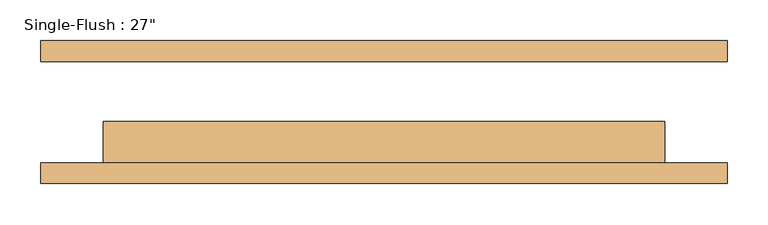
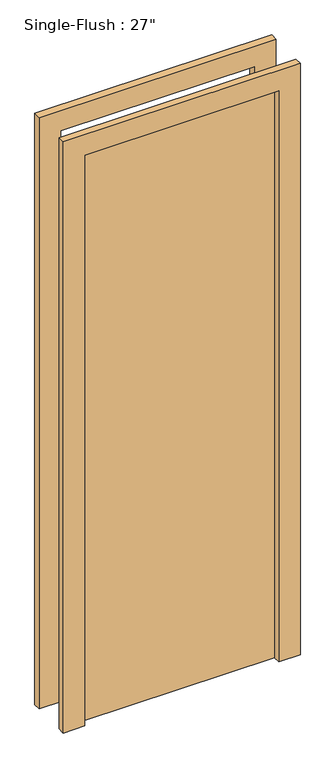
"""IFC4 building model written with IfcOpenShell, lengths in millimetres: door geometry."""

import ifcopenshell
import ifcopenshell.guid

model = None  # the IFC model being written
_history = None  # IfcOwnerHistory: only IFC2X3 demands one
_inside = {}  # id of a spatial element -> (the spatial element, [elements in it])
_under = {}  # id of a project, library or spatial element -> (it, [spatial elements below it])
_declared = {}  # id of a project -> (the project, [libraries it declares])
_typed = {}  # id of a type object -> (the type object, [elements of that type])
_made_of = {}  # id of a material, layer set ... -> (it, [elements and type objects made of it])


def new_model(schema):
    """Start an empty IFC model of exactly this schema.

    Asked for "IFC4X3", IfcOpenShell would pick the latest addendum, in which some entities
    have other attributes; the version numbers below select the first issue.
    IFC2X3 requires an IfcOwnerHistory on every rooted entity: one is made here for all.
    """
    global model, _history
    if schema == "IFC4X3":
        model = ifcopenshell.file(schema_version=(4, 3, 0, 0))
    else:
        model = ifcopenshell.file(schema=schema)
    _inside.clear()
    _under.clear()
    _declared.clear()
    _typed.clear()
    _made_of.clear()
    _history = None
    if model.schema == "IFC2X3":
        org = make("IfcOrganization", Name="unknown")
        user = make(
            "IfcPersonAndOrganization",
            ThePerson=make("IfcPerson", FamilyName="unknown"),
            TheOrganization=org,
        )
        app = make(
            "IfcApplication",
            ApplicationDeveloper=org,
            Version="unknown",
            ApplicationFullName="unknown",
            ApplicationIdentifier="unknown",
        )
        _history = make(
            "IfcOwnerHistory",
            OwningUser=user,
            OwningApplication=app,
            ChangeAction="ADDED",
            CreationDate=0,
        )
    return model


def make(cls, **values):
    """One entity of the class cls with the attributes given. An attribute that is None is left unset."""
    return model.create_entity(
        cls, **{name: value for name, value in values.items() if value is not None}
    )


def rooted(cls, **values):
    """An entity with a GlobalId (a new one), such as an element, a storey or a relation."""
    return make(cls, GlobalId=ifcopenshell.guid.new(), OwnerHistory=_history, **values)


def si_unit(unit_type, name, prefix=None):
    """IfcSIUnit, for example si_unit("LENGTHUNIT", "METRE", prefix="MILLI")."""
    return make("IfcSIUnit", UnitType=unit_type, Prefix=prefix, Name=name)


def assignment(units):
    """IfcUnitAssignment: the units of a project."""
    return None if units is None else make("IfcUnitAssignment", Units=units)


def point(xyz):
    """IfcCartesianPoint."""
    return None if xyz is None else make("IfcCartesianPoint", Coordinates=xyz)


def direction(xyz):
    """IfcDirection."""
    return None if xyz is None else make("IfcDirection", DirectionRatios=xyz)


def frame(location, z_axis=None, x_axis=None):
    """IfcAxis2Placement3D, a coordinate frame: its origin and axes. An axis left out is left unset."""
    return make(
        "IfcAxis2Placement3D",
        Location=point(location),
        Axis=direction(z_axis),
        RefDirection=direction(x_axis),
    )


def origin():
    """The frame at (0, 0, 0) with its axes left unset."""
    return frame((0.0, 0.0, 0.0))


def origin_with_axes():
    """The frame at (0, 0, 0) with the z axis (0, 0, 1) and the x axis (1, 0, 0) written out."""
    return frame((0.0, 0.0, 0.0), z_axis=(0.0, 0.0, 1.0), x_axis=(1.0, 0.0, 0.0))


def place(relative_to, where):
    """IfcLocalPlacement: puts the frame where relative to a parent placement (None: the world)."""
    return make(
        "IfcLocalPlacement", PlacementRelTo=relative_to, RelativePlacement=where
    )


def context(
    kind, dimensions, precision=None, world=None, true_north=None, identifier=None
):
    """IfcGeometricRepresentationContext, for example the 3D "Model" context."""
    return make(
        "IfcGeometricRepresentationContext",
        ContextIdentifier=identifier,
        ContextType=kind,
        CoordinateSpaceDimension=dimensions,
        Precision=precision,
        WorldCoordinateSystem=world,
        TrueNorth=true_north,
    )


def project(units=None, contexts=None):
    """IfcProject with its units and contexts."""
    return rooted(
        "IfcProject",
        Name="project",
        RepresentationContexts=contexts,
        UnitsInContext=assignment(units),
    )


def spatial(cls, under=None, at=None, **own):
    """A site, building, storey or space (cls), placed at a placement, below another one or the project."""
    s = rooted(cls, ObjectPlacement=at, **own)
    if under is not None:
        _under.setdefault(under.id(), (under, []))[1].append(s)
    return s


def polyline(points):
    """IfcPolyline through the points."""
    return make("IfcPolyline", Points=[point(p) for p in points])


def outline(outer, holes=None, kind="AREA"):
    """IfcArbitraryClosedProfileDef: a profile drawn as a closed curve; with holes, ...WithVoids."""
    if holes is None:
        return make("IfcArbitraryClosedProfileDef", ProfileType=kind, OuterCurve=outer)
    return make(
        "IfcArbitraryProfileDefWithVoids",
        ProfileType=kind,
        OuterCurve=outer,
        InnerCurves=holes,
    )


def extrude(swept, where, along, depth):
    """IfcExtrudedAreaSolid: the profile swept, set in the frame where, extruded along a direction by depth."""
    return make(
        "IfcExtrudedAreaSolid",
        SweptArea=swept,
        Position=where,
        ExtrudedDirection=direction(along),
        Depth=depth,
    )


def shape(context_of_items, identifier, shape_type, items):
    """IfcShapeRepresentation: the items that make up one representation, for example the "Body"."""
    return make(
        "IfcShapeRepresentation",
        ContextOfItems=context_of_items,
        RepresentationIdentifier=identifier,
        RepresentationType=shape_type,
        Items=items,
    )


def source(mapping_origin, context_of_items, identifier, shape_type, items):
    """IfcRepresentationMap: a shape defined once, which mapped items show again and again."""
    return make(
        "IfcRepresentationMap",
        MappingOrigin=mapping_origin,
        MappedRepresentation=shape(context_of_items, identifier, shape_type, items),
    )


def transform(
    local_origin,
    x_axis=None,
    y_axis=None,
    z_axis=None,
    scale=None,
    scale2=None,
    scale3=None,
    uniform=True,
):
    """IfcCartesianTransformationOperator3D, or its non-uniform kind. x_axis, y_axis, z_axis: its Axis1, 2, 3."""
    if uniform:
        return make(
            "IfcCartesianTransformationOperator3D",
            Axis1=direction(x_axis),
            Axis2=direction(y_axis),
            LocalOrigin=point(local_origin),
            Scale=scale,
            Axis3=direction(z_axis),
        )
    return make(
        "IfcCartesianTransformationOperator3DnonUniform",
        Axis1=direction(x_axis),
        Axis2=direction(y_axis),
        LocalOrigin=point(local_origin),
        Scale=scale,
        Axis3=direction(z_axis),
        Scale2=scale2,
        Scale3=scale3,
    )


def mapped(mapping_source, mapping_target):
    """IfcMappedItem: shows the shape of a source again, moved by a transform."""
    return make(
        "IfcMappedItem", MappingSource=mapping_source, MappingTarget=mapping_target
    )


def made_of(thing, what):
    """Note that an element or type object is made of a material, layer set ...; save() writes the relation."""
    if what is not None:
        _made_of.setdefault(what.id(), (what, []))[1].append(thing)
    return thing


def element(
    cls,
    number,
    at=None,
    inside=None,
    cuts=None,
    type_object=None,
    material=None,
    context=None,
    identifier="Body",
    shape_type=None,
    held_by="IfcProductDefinitionShape",
    body=None,
    shapes=None,
    **own,
):
    """One element of the class cls, such as IfcWall. Its Tag is "e" and its number.

    at: its placement. inside: the storey or other place that contains it. cuts: it is an
    opening in that element (IfcRelVoidsElement). A single representation is given by context,
    identifier, shape_type and body (its items); several are given by shapes. held_by: the class
    of the entity that holds the representations. save() writes the other relations.
    """
    e = rooted(cls, Tag="e%d" % number, ObjectPlacement=at, **own)
    if body is not None:
        shapes = [shape(context, identifier, shape_type, body)]
    if shapes is not None:
        e.Representation = make(held_by, Representations=shapes)
    if inside is not None:
        _inside.setdefault(inside.id(), (inside, []))[1].append(e)
    if cuts is not None:
        rooted(
            "IfcRelVoidsElement", RelatingBuildingElement=cuts, RelatedOpeningElement=e
        )
    if type_object is not None:
        _typed.setdefault(type_object.id(), (type_object, []))[1].append(e)
    return made_of(e, material)


def aggregate(whole, parts):
    """IfcRelAggregates: a whole, such as a stair, and the parts it consists of."""
    return rooted("IfcRelAggregates", RelatingObject=whole, RelatedObjects=parts)


def save(model, path):
    """Write the relations noted so far, then the file.

    IfcRelAggregates (storeys below a building ...), IfcRelContainedInSpatialStructure (elements
    in a storey), IfcRelDefinesByType, IfcRelAssociatesMaterial and IfcRelDeclares: one each for
    every whole, place, type object, material and project.
    """
    for whole, parts in _under.values():
        aggregate(whole, parts)
    for where, things in _inside.values():
        rooted(
            "IfcRelContainedInSpatialStructure",
            RelatedElements=things,
            RelatingStructure=where,
        )
    for kind, things in _typed.values():
        rooted("IfcRelDefinesByType", RelatedObjects=things, RelatingType=kind)
    for what, things in _made_of.values():
        rooted("IfcRelAssociatesMaterial", RelatedObjects=things, RelatingMaterial=what)
    for by, libraries in _declared.values():
        rooted("IfcRelDeclares", RelatingContext=by, RelatedDefinitions=libraries)
    model.write(path)


def door_ae44b9d4(model_context):
    return source(origin(), model_context, "Body", "SweptSolid", [
        extrude(outline(polyline([(2209.8, -419.1), (0.0, -419.1), (0.0, -342.9), (2133.6, -342.9), (2133.6, 342.9), (0.0, 342.9), (0.0, 419.1), (2209.8, 419.1), (2209.8, -419.1)])), frame((0.0, -87.3125, 0.0), z_axis=(0.0, 1.0, 0.0), x_axis=(0.0, 0.0, 1.0)), (0.0, 0.0, 1.0), 25.4),
        extrude(outline(polyline([(2209.8, 419.1), (2209.8, -419.1), (0.0, -419.1), (0.0, -342.9), (2133.6, -342.9), (2133.6, 342.9), (0.0, 342.9), (0.0, 419.1), (2209.8, 419.1)])), frame((0.0, 61.9125, 0.0), z_axis=(0.0, 1.0, 0.0), x_axis=(0.0, 0.0, 1.0)), (0.0, 0.0, 1.0), 25.4),
        extrude(outline(polyline([(342.9, -11.1125), (342.9, -61.9125), (-342.9, -61.9125), (-342.9, -11.1125), (342.9, -11.1125)])), origin_with_axes(), (0.0, 0.0, 1.0), 2133.6),
    ])


if __name__ == "__main__":
    model = new_model("IFC4")
    model_context = context("Model", 3, world=origin())
    ifc_project = project(units=[si_unit("LENGTHUNIT", "METRE", prefix="MILLI")], contexts=[model_context])
    site = spatial("IfcSite", under=ifc_project)
    building = spatial("IfcBuilding", under=site)
    placement = place(None, origin())
    door_shape = door_ae44b9d4(model_context)
    element("IfcDoor", 1, ObjectType="Single-Flush : 27\"", at=placement, inside=building, context=model_context, shape_type="MappedRepresentation", body=[
        mapped(door_shape, transform((0.0, 0.0, 0.0), x_axis=(1.0, 0.0, 0.0), y_axis=(0.0, 1.0, 0.0), z_axis=(0.0, 0.0, 1.0))),
    ])
    save(model, "model.ifc")

# Revit data of these elements
# Type "Single-Flush : 27\""
#   Type Mark = "55"
#   Construction Type Id = "MDOOR"
#   Assembly Code = "C1020"
#   Analytic Construction = "Metal"
#   Thickness = 0' - 2"
#   Heat Transfer Coefficient (U) = 3.7021 W/(m²·K)
#   Height = 7' - 0"
#   Trim Projection Ext = 0' - 1"
#   Trim Projection Int = 0' - 1"
#   Trim Width = 0' - 3"
#   Width = 2' - 3"
#   Door Material = Door - Panel
#   Frame Material = Door - Frame
#   Visual Light Transmittance = 0
#   Solar Heat Gain Coefficient = 0
#   Function = (empty or 0)
#   Wall Closure = (empty or 0)
# Element 1 (IfcDoor, "Single-Flush : 27\"")
#   Materials on its faces: "Door - Frame", "Door - Panel"
# Materials
#   "Door - Panel": class "Wood", colour RGB 210 159 95, transparency 0
#   "Door - Frame": class "Miscellaneous", colour RGB 118 70 51, transparency 0
